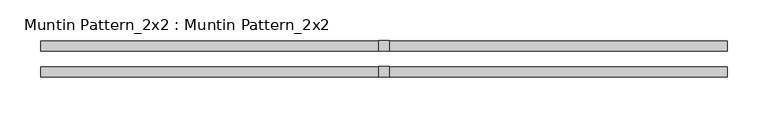
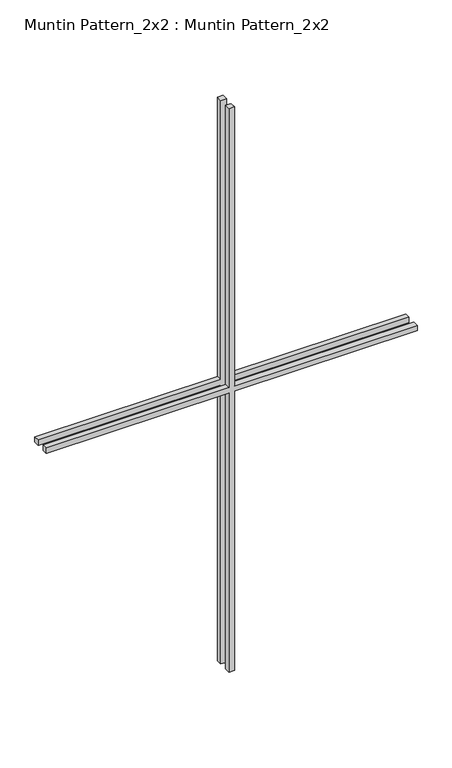
"""IFC4 building model written with IfcOpenShell, lengths in millimetres: proxy geometry, Muntin Pattern_2x2 : Muntin Pattern_2x2."""

from ifc_helpers import new_model, si_unit, frame, origin, place, context, project, spatial, polyline, outline, extrude, source, transform, mapped, element, save


def muntin_pattern_2x2_muntin_pattern_2x2_809937e0(model_context):
    return source(origin(), model_context, "Body", "SweptSolid", [
        extrude(outline(polyline([(679.45, -6.35), (679.45, -419.1), (666.75, -419.1), (666.75, -6.35), (0.0, -6.35), (0.0, 6.35), (666.75, 6.35), (666.75, 419.1), (679.45, 419.1), (679.45, 6.35), (1346.2, 6.35), (1346.2, -6.35), (679.45, -6.35)])), frame((0.0, -22.225, 0.0), z_axis=(0.0, 1.0, 0.0), x_axis=(0.0, 0.0, 1.0)), (0.0, 0.0, 1.0), 12.7),
        extrude(outline(polyline([(679.45, -6.35), (679.45, -419.1), (666.75, -419.1), (666.75, -6.35), (0.0, -6.35), (0.0, 6.35), (666.75, 6.35), (666.75, 419.1), (679.45, 419.1), (679.45, 6.35), (1346.2, 6.35), (1346.2, -6.35), (679.45, -6.35)])), frame((0.0, 9.525, 0.0), z_axis=(0.0, 1.0, 0.0), x_axis=(0.0, 0.0, 1.0)), (0.0, 0.0, 1.0), 12.7),
    ])


if __name__ == "__main__":
    model = new_model("IFC4")
    model_context = context("Model", 3, world=origin())
    ifc_project = project(units=[si_unit("LENGTHUNIT", "METRE", prefix="MILLI")], contexts=[model_context])
    site = spatial("IfcSite", under=ifc_project)
    building = spatial("IfcBuilding", under=site)
    placement = place(None, origin())
    muntin_pattern_2x2_muntin_pattern_2x2_shape = muntin_pattern_2x2_muntin_pattern_2x2_809937e0(model_context)
    element("IfcBuildingElementProxy", 1, Name="Muntin Pattern_2x2 : Muntin Pattern_2x2", ObjectType="Muntin Pattern_2x2 : Muntin Pattern_2x2", at=placement, inside=building, context=model_context, shape_type="MappedRepresentation", body=[
        mapped(muntin_pattern_2x2_muntin_pattern_2x2_shape, transform((0.0, 0.0, 0.0), x_axis=(1.0, 0.0, 0.0), y_axis=(0.0, 1.0, 0.0), z_axis=(0.0, 0.0, 1.0))),
    ])
    save(model, "model.ifc")

# Revit data of these elements
# Type "Muntin Pattern_2x2 : Muntin Pattern_2x2"
#   Width [instance default] = 4' - 0"
#   Thickness = 0' - 0 1/2"
#   Height [instance default] = 4' - 0"
#   Distance = 0' - 0 3/4"
#   Interior Material [instance default] = none
#   Exterior Material [instance default] = none
#   Default Elevation = 0
# Element 1 (IfcBuildingElementProxy, "Muntin Pattern_2x2 : Muntin Pattern_2x2")
#   Width = 2' - 9"
#   Height = 4' - 5"
#   Interior Material = Wood - Stained
#   Exterior Material = Clad - White
#   Materials on its faces: "Clad - White", "Wood - Stained"
# Materials
#   "Clad - White": class "Wood", colour RGB 242 242 238, transparency 0, Cost = 0
#   "Wood - Stained": class "Wood", colour RGB 224 178 126, transparency 0, Cost = 0
